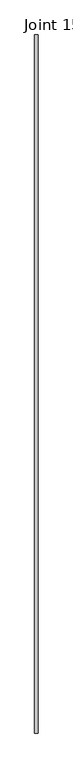
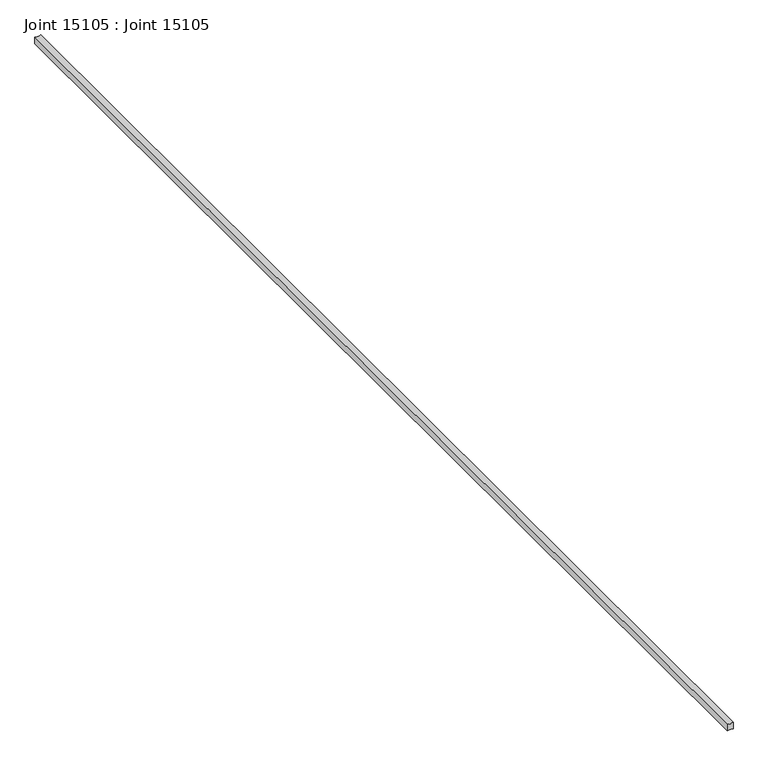
"""IFC4 building model written with IfcOpenShell, lengths in millimetres: proxy geometry, Joint 15105 : Joint 15105."""

import ifcopenshell
import ifcopenshell.guid

model = None  # the IFC model being written
_history = None  # IfcOwnerHistory: only IFC2X3 demands one
_inside = {}  # id of a spatial element -> (the spatial element, [elements in it])
_under = {}  # id of a project, library or spatial element -> (it, [spatial elements below it])
_declared = {}  # id of a project -> (the project, [libraries it declares])
_typed = {}  # id of a type object -> (the type object, [elements of that type])
_made_of = {}  # id of a material, layer set ... -> (it, [elements and type objects made of it])


def new_model(schema):
    """Start an empty IFC model of exactly this schema.

    Asked for "IFC4X3", IfcOpenShell would pick the latest addendum, in which some entities
    have other attributes; the version numbers below select the first issue.
    IFC2X3 requires an IfcOwnerHistory on every rooted entity: one is made here for all.
    """
    global model, _history
    if schema == "IFC4X3":
        model = ifcopenshell.file(schema_version=(4, 3, 0, 0))
    else:
        model = ifcopenshell.file(schema=schema)
    _inside.clear()
    _under.clear()
    _declared.clear()
    _typed.clear()
    _made_of.clear()
    _history = None
    if model.schema == "IFC2X3":
        org = make("IfcOrganization", Name="unknown")
        user = make(
            "IfcPersonAndOrganization",
            ThePerson=make("IfcPerson", FamilyName="unknown"),
            TheOrganization=org,
        )
        app = make(
            "IfcApplication",
            ApplicationDeveloper=org,
            Version="unknown",
            ApplicationFullName="unknown",
            ApplicationIdentifier="unknown",
        )
        _history = make(
            "IfcOwnerHistory",
            OwningUser=user,
            OwningApplication=app,
            ChangeAction="ADDED",
            CreationDate=0,
        )
    return model


def make(cls, **values):
    """One entity of the class cls with the attributes given. An attribute that is None is left unset."""
    return model.create_entity(
        cls, **{name: value for name, value in values.items() if value is not None}
    )


def rooted(cls, **values):
    """An entity with a GlobalId (a new one), such as an element, a storey or a relation."""
    return make(cls, GlobalId=ifcopenshell.guid.new(), OwnerHistory=_history, **values)


def si_unit(unit_type, name, prefix=None):
    """IfcSIUnit, for example si_unit("LENGTHUNIT", "METRE", prefix="MILLI")."""
    return make("IfcSIUnit", UnitType=unit_type, Prefix=prefix, Name=name)


def assignment(units):
    """IfcUnitAssignment: the units of a project."""
    return None if units is None else make("IfcUnitAssignment", Units=units)


def point(xyz):
    """IfcCartesianPoint."""
    return None if xyz is None else make("IfcCartesianPoint", Coordinates=xyz)


def direction(xyz):
    """IfcDirection."""
    return None if xyz is None else make("IfcDirection", DirectionRatios=xyz)


def frame(location, z_axis=None, x_axis=None):
    """IfcAxis2Placement3D, a coordinate frame: its origin and axes. An axis left out is left unset."""
    return make(
        "IfcAxis2Placement3D",
        Location=point(location),
        Axis=direction(z_axis),
        RefDirection=direction(x_axis),
    )


def frame_2d(location, x_axis=None):
    """IfcAxis2Placement2D, a coordinate frame in the plane: its origin and x axis."""
    return make(
        "IfcAxis2Placement2D", Location=point(location), RefDirection=direction(x_axis)
    )


def origin():
    """The frame at (0, 0, 0) with its axes left unset."""
    return frame((0.0, 0.0, 0.0))


def place(relative_to, where):
    """IfcLocalPlacement: puts the frame where relative to a parent placement (None: the world)."""
    return make(
        "IfcLocalPlacement", PlacementRelTo=relative_to, RelativePlacement=where
    )


def context(
    kind, dimensions, precision=None, world=None, true_north=None, identifier=None
):
    """IfcGeometricRepresentationContext, for example the 3D "Model" context."""
    return make(
        "IfcGeometricRepresentationContext",
        ContextIdentifier=identifier,
        ContextType=kind,
        CoordinateSpaceDimension=dimensions,
        Precision=precision,
        WorldCoordinateSystem=world,
        TrueNorth=true_north,
    )


def project(units=None, contexts=None):
    """IfcProject with its units and contexts."""
    return rooted(
        "IfcProject",
        Name="project",
        RepresentationContexts=contexts,
        UnitsInContext=assignment(units),
    )


def spatial(cls, under=None, at=None, **own):
    """A site, building, storey or space (cls), placed at a placement, below another one or the project."""
    s = rooted(cls, ObjectPlacement=at, **own)
    if under is not None:
        _under.setdefault(under.id(), (under, []))[1].append(s)
    return s


def polyline(points):
    """IfcPolyline through the points."""
    return make("IfcPolyline", Points=[point(p) for p in points])


def circle_curve(where, radius):
    """IfcCircle in the frame where."""
    return make("IfcCircle", Position=where, Radius=radius)


def trimmed(basis, trim1, trim2, sense, master):
    """IfcTrimmedCurve: the piece of a basis curve between two trims."""
    return make(
        "IfcTrimmedCurve",
        BasisCurve=basis,
        Trim1=trim1,
        Trim2=trim2,
        SenseAgreement=sense,
        MasterRepresentation=master,
    )


def segment(curve, same_sense, transition):
    """IfcCompositeCurveSegment."""
    return make(
        "IfcCompositeCurveSegment",
        Transition=transition,
        SameSense=same_sense,
        ParentCurve=curve,
    )


def composite_curve(segments, self_intersect=None):
    """IfcCompositeCurve: segments joined end to end."""
    return make("IfcCompositeCurve", Segments=segments, SelfIntersect=self_intersect)


def outline(outer, holes=None, kind="AREA"):
    """IfcArbitraryClosedProfileDef: a profile drawn as a closed curve; with holes, ...WithVoids."""
    if holes is None:
        return make("IfcArbitraryClosedProfileDef", ProfileType=kind, OuterCurve=outer)
    return make(
        "IfcArbitraryProfileDefWithVoids",
        ProfileType=kind,
        OuterCurve=outer,
        InnerCurves=holes,
    )


def extrude(swept, where, along, depth):
    """IfcExtrudedAreaSolid: the profile swept, set in the frame where, extruded along a direction by depth."""
    return make(
        "IfcExtrudedAreaSolid",
        SweptArea=swept,
        Position=where,
        ExtrudedDirection=direction(along),
        Depth=depth,
    )


def shape(context_of_items, identifier, shape_type, items):
    """IfcShapeRepresentation: the items that make up one representation, for example the "Body"."""
    return make(
        "IfcShapeRepresentation",
        ContextOfItems=context_of_items,
        RepresentationIdentifier=identifier,
        RepresentationType=shape_type,
        Items=items,
    )


def source(mapping_origin, context_of_items, identifier, shape_type, items):
    """IfcRepresentationMap: a shape defined once, which mapped items show again and again."""
    return make(
        "IfcRepresentationMap",
        MappingOrigin=mapping_origin,
        MappedRepresentation=shape(context_of_items, identifier, shape_type, items),
    )


def transform(
    local_origin,
    x_axis=None,
    y_axis=None,
    z_axis=None,
    scale=None,
    scale2=None,
    scale3=None,
    uniform=True,
):
    """IfcCartesianTransformationOperator3D, or its non-uniform kind. x_axis, y_axis, z_axis: its Axis1, 2, 3."""
    if uniform:
        return make(
            "IfcCartesianTransformationOperator3D",
            Axis1=direction(x_axis),
            Axis2=direction(y_axis),
            LocalOrigin=point(local_origin),
            Scale=scale,
            Axis3=direction(z_axis),
        )
    return make(
        "IfcCartesianTransformationOperator3DnonUniform",
        Axis1=direction(x_axis),
        Axis2=direction(y_axis),
        LocalOrigin=point(local_origin),
        Scale=scale,
        Axis3=direction(z_axis),
        Scale2=scale2,
        Scale3=scale3,
    )


def mapped(mapping_source, mapping_target):
    """IfcMappedItem: shows the shape of a source again, moved by a transform."""
    return make(
        "IfcMappedItem", MappingSource=mapping_source, MappingTarget=mapping_target
    )


def made_of(thing, what):
    """Note that an element or type object is made of a material, layer set ...; save() writes the relation."""
    if what is not None:
        _made_of.setdefault(what.id(), (what, []))[1].append(thing)
    return thing


def element(
    cls,
    number,
    at=None,
    inside=None,
    cuts=None,
    type_object=None,
    material=None,
    context=None,
    identifier="Body",
    shape_type=None,
    held_by="IfcProductDefinitionShape",
    body=None,
    shapes=None,
    **own,
):
    """One element of the class cls, such as IfcWall. Its Tag is "e" and its number.

    at: its placement. inside: the storey or other place that contains it. cuts: it is an
    opening in that element (IfcRelVoidsElement). A single representation is given by context,
    identifier, shape_type and body (its items); several are given by shapes. held_by: the class
    of the entity that holds the representations. save() writes the other relations.
    """
    e = rooted(cls, Tag="e%d" % number, ObjectPlacement=at, **own)
    if body is not None:
        shapes = [shape(context, identifier, shape_type, body)]
    if shapes is not None:
        e.Representation = make(held_by, Representations=shapes)
    if inside is not None:
        _inside.setdefault(inside.id(), (inside, []))[1].append(e)
    if cuts is not None:
        rooted(
            "IfcRelVoidsElement", RelatingBuildingElement=cuts, RelatedOpeningElement=e
        )
    if type_object is not None:
        _typed.setdefault(type_object.id(), (type_object, []))[1].append(e)
    return made_of(e, material)


def aggregate(whole, parts):
    """IfcRelAggregates: a whole, such as a stair, and the parts it consists of."""
    return rooted("IfcRelAggregates", RelatingObject=whole, RelatedObjects=parts)


def save(model, path):
    """Write the relations noted so far, then the file.

    IfcRelAggregates (storeys below a building ...), IfcRelContainedInSpatialStructure (elements
    in a storey), IfcRelDefinesByType, IfcRelAssociatesMaterial and IfcRelDeclares: one each for
    every whole, place, type object, material and project.
    """
    for whole, parts in _under.values():
        aggregate(whole, parts)
    for where, things in _inside.values():
        rooted(
            "IfcRelContainedInSpatialStructure",
            RelatedElements=things,
            RelatingStructure=where,
        )
    for kind, things in _typed.values():
        rooted("IfcRelDefinesByType", RelatedObjects=things, RelatingType=kind)
    for what, things in _made_of.values():
        rooted("IfcRelAssociatesMaterial", RelatedObjects=things, RelatingMaterial=what)
    for by, libraries in _declared.values():
        rooted("IfcRelDeclares", RelatingContext=by, RelatedDefinitions=libraries)
    model.write(path)


def joint_15105_joint_15105_0664364a(model_context):
    return source(origin(), model_context, "Body", "SweptSolid", [
        extrude(outline(composite_curve([segment(trimmed(circle_curve(frame_2d((40345.8971102, -980.0560021)), 11.4720018), [point((40335.8421875, -974.5328369))], [point((40335.3398438, -984.5449829))], True, "CARTESIAN"), True, "CONTINUOUS"), segment(polyline([(40335.3398438, -984.5449829), (40323.640625, -984.5449829)]), True, "CONTINUOUS"), segment(trimmed(circle_curve(frame_2d((40313.8157186, -979.5389099)), 11.0267653), [point((40323.640625, -984.5449829))], [point((40323.640625, -974.5328369))], True, "CARTESIAN"), True, "CONTINUOUS"), segment(polyline([(40323.640625, -974.5328369), (40335.8421875, -974.5328369)]), True, "CONTINUOUS")], self_intersect=False)), frame((0.0, -1052.8906574, 0.0), z_axis=(0.0, 1.0, 0.0), x_axis=(0.0, 0.0, 1.0)), (0.0, 0.0, 1.0), 2000.0),
    ])


if __name__ == "__main__":
    model = new_model("IFC4")
    model_context = context("Model", 3, world=origin())
    ifc_project = project(units=[si_unit("LENGTHUNIT", "METRE", prefix="MILLI")], contexts=[model_context])
    site = spatial("IfcSite", under=ifc_project)
    building = spatial("IfcBuilding", under=site)
    placement = place(None, origin())
    joint_15105_joint_15105_shape = joint_15105_joint_15105_0664364a(model_context)
    element("IfcBuildingElementProxy", 1, Name="Joint 15105 : Joint 15105", ObjectType="Joint 15105 : Joint 15105", at=placement, inside=building, context=model_context, shape_type="MappedRepresentation", body=[
        mapped(joint_15105_joint_15105_shape, transform((0.0, 0.0, 0.0), x_axis=(1.0, 0.0, 0.0), y_axis=(0.0, 1.0, 0.0), z_axis=(0.0, 0.0, 1.0))),
    ])
    save(model, "model.ifc")

# Revit data of these elements
# Type "Joint 15105 : Joint 15105"
#   NameOverride = "Joint"
# Element 1 (IfcBuildingElementProxy, "Joint 15105 : Joint 15105")
#   Materials on its faces: "SEALANT"
# Materials
#   "SEALANT": class "Unassigned", colour RGB 142 225 148, transparency 0
